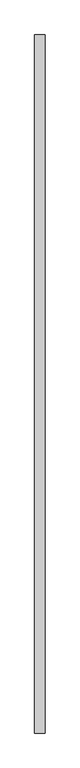
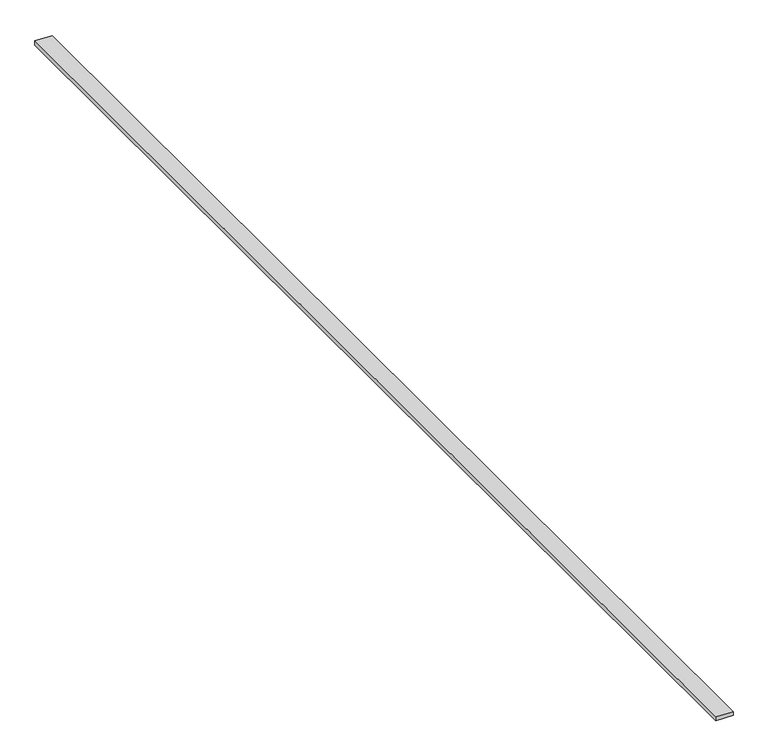
"""IFC4 building model written with IfcOpenShell, lengths in millimetres: proxy geometry, Generic Models 7:Generic Models 1:337419:Generic Models 1:337419 : Generic Models 7:Generic Models 1:337419:30 : Generic Models 7:Generic Models 1:337419:Generic Models 1:337419 : Generic Models 7:Generic Models 1:337419:301336."""

from ifc_helpers import new_model, si_unit, frame, origin, place, context, project, spatial, polyline, outline, extrude, source, transform, mapped, element, save


def generic_models_b355f30f(model_context):
    return source(origin(), model_context, "Body", "SweptSolid", [
        extrude(outline(polyline([(6128.940625, 560321.211724), (6128.940625, 560505.361724), (6169.4995614, 560505.361724), (6179.1504539, 560321.211724), (6128.940625, 560321.211724)])), frame((0.0, -578946.7163842, 0.0), z_axis=(0.0, 1.0, 0.0), x_axis=(0.0, 0.0, 1.0)), (0.0, 0.0, 1.0), 12477.75),
    ])


if __name__ == "__main__":
    model = new_model("IFC4")
    model_context = context("Model", 3, world=origin())
    ifc_project = project(units=[si_unit("LENGTHUNIT", "METRE", prefix="MILLI")], contexts=[model_context])
    site = spatial("IfcSite", under=ifc_project)
    building = spatial("IfcBuilding", under=site)
    placement = place(None, origin())
    generic_models_shape = generic_models_b355f30f(model_context)
    element("IfcBuildingElementProxy", 1, Name="Generic Models 7:Generic Models 1:337419:Generic Models 1:337419 : Generic Models 7:Generic Models 1:337419:30 : Generic Models 7:Generic Models 1:337419:Generic Models 1:337419 : Generic Models 7:Generic Models 1:337419:301336", ObjectType="Generic Models 7:Generic Models 1:337419:Generic Models 1:337419 : Generic Models 7:Generic Models 1:337419:30 : Generic Models 7:Generic Models 1:337419:Generic Models 1:337419 : Generic Models 7:Generic Models 1:337419:301336", at=placement, inside=building, context=model_context, shape_type="MappedRepresentation", body=[
        mapped(generic_models_shape, transform((0.0, 0.0, 0.0), x_axis=(1.0, 0.0, 0.0), y_axis=(0.0, 1.0, 0.0), z_axis=(0.0, 0.0, 1.0))),
    ])
    save(model, "model.ifc")

# Revit data of these elements
# Type "Generic Models 7:Generic Models 1:337419:Generic Models 1:337419 : Generic Models 7:Generic Models 1:337419:30 : Generic Models 7:Generic Models 1:337419:Generic Models 1:337419 : Generic Models 7:Generic Models 1:337419:301336"
#   NameOverride = "Generic Models 7:Generic Models 1:337419:Generic Models 1:337419 : Generic Models 7:Generic Models 1:337419:301336"
#   ObjectTypeOverride = "Generic Models 1:337419 : Generic Models 7:Generic Models 1:337419"
#   Reference = "Generic Models 1"
#   Tag = "301336"
# Element 1 (IfcBuildingElementProxy, "Generic Models 7:Generic Models 1:337419:Generic Models 1:337419 : Generic Models 7:Generic Models 1:337419:30 : Generic Models 7:Generic Models 1:337419:Generic Models 1:337419 : Generic Models 7:Generic Models 1:337419:301336")
#   Materials on its faces: "FIRE RETARDTANT WOOD BLOCKING - SIZE AS NECESSARY"
# Materials
#   "FIRE RETARDTANT WOOD BLOCKING - SIZE AS NECESSARY": class "Wood", colour RGB 144 113 62, transparency 0, Description = "Pinus Echinata", Cost = 0
